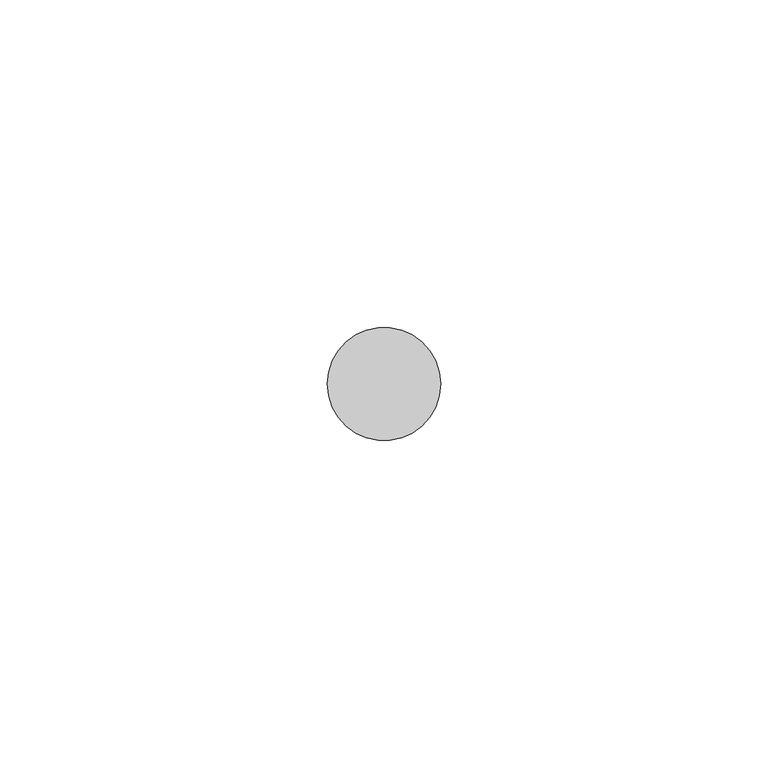
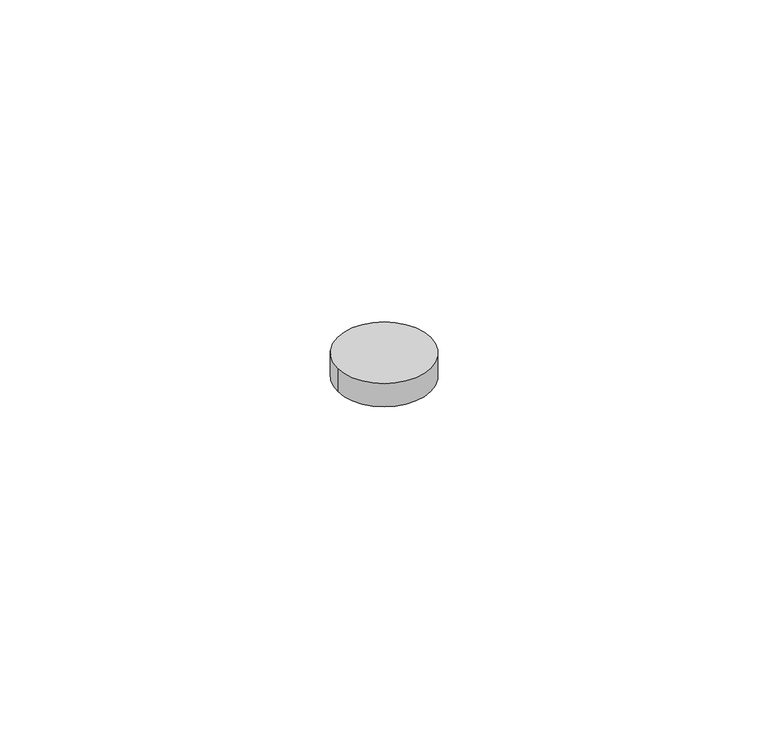
"""IFC4 building model written with IfcOpenShell, lengths in millimetres: proxy geometry, Hinge Pin Keeper9 : Hinge Pin Keeper."""

from ifc_helpers import new_model, si_unit, point, frame, frame_2d, origin, place, context, project, spatial, circle_curve, trimmed, segment, composite_curve, outline, extrude, source, transform, mapped, element, save


def generic_models_21f6d7d6(model_context):
    return source(origin(), model_context, "Body", "SweptSolid", [
        extrude(outline(composite_curve([segment(trimmed(circle_curve(frame_2d((587319.1320739, -536310.3652841)), 8.6534625), [point((587310.4786114, -536310.3652841))], [point((587327.7855364, -536310.3652841))], False, "CARTESIAN"), True, "CONTINUOUS"), segment(trimmed(circle_curve(frame_2d((587319.1320739, -536310.3652841)), 8.6534625), [point((587327.7855364, -536310.3652841))], [point((587310.4786114, -536310.3652841))], False, "CARTESIAN"), True, "CONTINUOUS")], self_intersect=False)), frame((0.0, 0.0, 458.9859375), z_axis=(0.0, 0.0, 1.0), x_axis=(1.0, 0.0, 0.0)), (0.0, 0.0, 1.0), 4.5640625),
    ])


if __name__ == "__main__":
    model = new_model("IFC4")
    model_context = context("Model", 3, world=origin())
    ifc_project = project(units=[si_unit("LENGTHUNIT", "METRE", prefix="MILLI")], contexts=[model_context])
    site = spatial("IfcSite", under=ifc_project)
    building = spatial("IfcBuilding", under=site)
    placement = place(None, origin())
    generic_models_shape = generic_models_21f6d7d6(model_context)
    element("IfcBuildingElementProxy", 1, Name="Hinge Pin Keeper9 : Hinge Pin Keeper", ObjectType="Hinge Pin Keeper9 : Hinge Pin Keeper", at=placement, inside=building, context=model_context, shape_type="MappedRepresentation", body=[
        mapped(generic_models_shape, transform((0.0, 0.0, 0.0), x_axis=(1.0, 0.0, 0.0), y_axis=(0.0, 1.0, 0.0), z_axis=(0.0, 0.0, 1.0))),
    ])
    save(model, "model.ifc")

# Revit data of these elements
# Element 1 (IfcBuildingElementProxy, "Hinge Pin Keeper9 : Hinge Pin Keeper")
#   Materials on its faces: "6\"X6\" WELD-ON STL BUTT HINGE"
# Materials
#   "6\"X6\" WELD-ON STL BUTT HINGE": class "Metal", colour RGB 189 187 185, transparency 0, Description = "Carbon steel", Cost = 0
